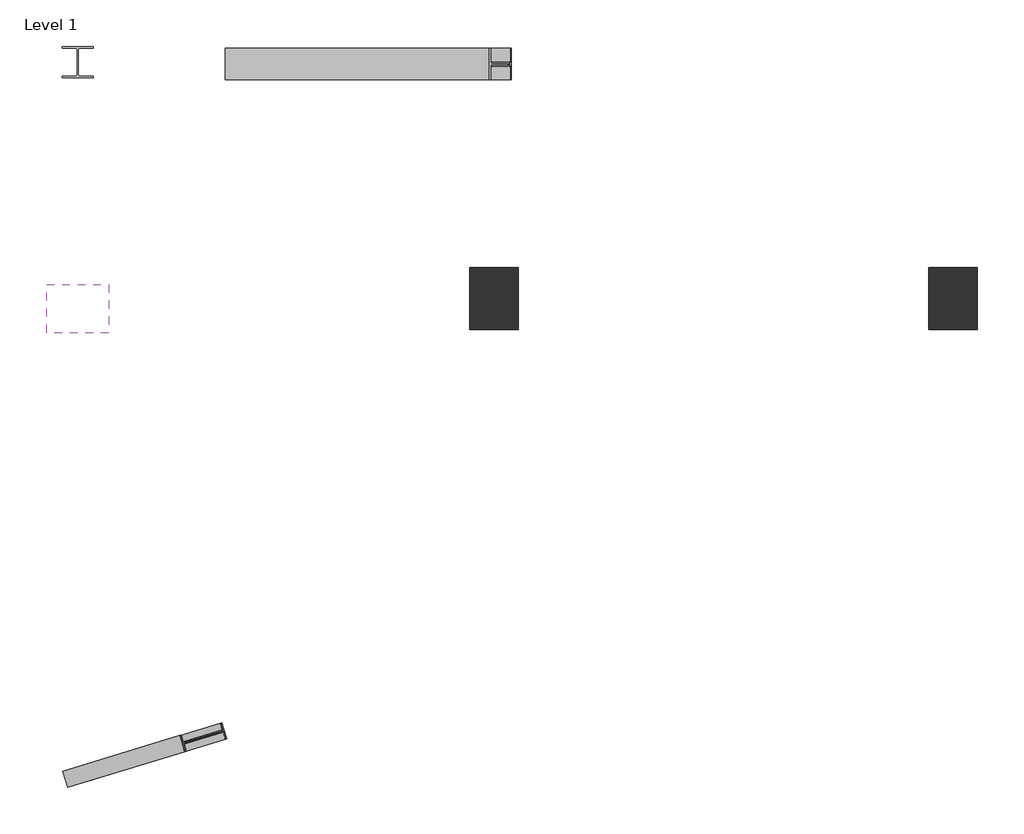
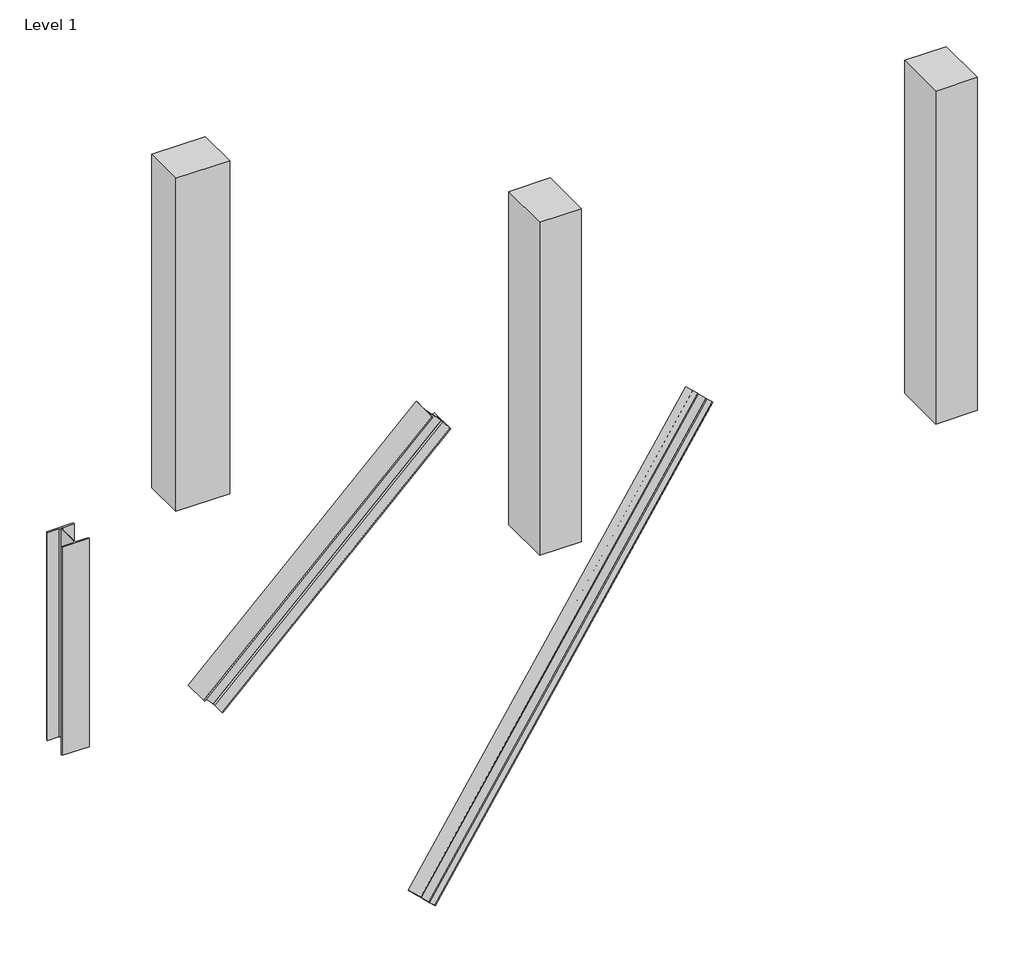
# One storey: 5 columns, 1 beam.
"""IFC4 building model written with IfcOpenShell, lengths in millimetres."""

import ifcopenshell
import ifcopenshell.guid

model = None  # the IFC model being written
_history = None  # IfcOwnerHistory: only IFC2X3 demands one
_inside = {}  # id of a spatial element -> (the spatial element, [elements in it])
_under = {}  # id of a project, library or spatial element -> (it, [spatial elements below it])
_declared = {}  # id of a project -> (the project, [libraries it declares])
_typed = {}  # id of a type object -> (the type object, [elements of that type])
_made_of = {}  # id of a material, layer set ... -> (it, [elements and type objects made of it])


def new_model(schema):
    """Start an empty IFC model of exactly this schema.

    Asked for "IFC4X3", IfcOpenShell would pick the latest addendum, in which some entities
    have other attributes; the version numbers below select the first issue.
    IFC2X3 requires an IfcOwnerHistory on every rooted entity: one is made here for all.
    """
    global model, _history
    if schema == "IFC4X3":
        model = ifcopenshell.file(schema_version=(4, 3, 0, 0))
    else:
        model = ifcopenshell.file(schema=schema)
    _inside.clear()
    _under.clear()
    _declared.clear()
    _typed.clear()
    _made_of.clear()
    _history = None
    if model.schema == "IFC2X3":
        org = make("IfcOrganization", Name="unknown")
        user = make(
            "IfcPersonAndOrganization",
            ThePerson=make("IfcPerson", FamilyName="unknown"),
            TheOrganization=org,
        )
        app = make(
            "IfcApplication",
            ApplicationDeveloper=org,
            Version="unknown",
            ApplicationFullName="unknown",
            ApplicationIdentifier="unknown",
        )
        _history = make(
            "IfcOwnerHistory",
            OwningUser=user,
            OwningApplication=app,
            ChangeAction="ADDED",
            CreationDate=0,
        )
    return model


def make(cls, **values):
    """One entity of the class cls with the attributes given. An attribute that is None is left unset."""
    return model.create_entity(
        cls, **{name: value for name, value in values.items() if value is not None}
    )


def rooted(cls, **values):
    """An entity with a GlobalId (a new one), such as an element, a storey or a relation."""
    return make(cls, GlobalId=ifcopenshell.guid.new(), OwnerHistory=_history, **values)


def si_unit(unit_type, name, prefix=None):
    """IfcSIUnit, for example si_unit("LENGTHUNIT", "METRE", prefix="MILLI")."""
    return make("IfcSIUnit", UnitType=unit_type, Prefix=prefix, Name=name)


def assignment(units):
    """IfcUnitAssignment: the units of a project."""
    return None if units is None else make("IfcUnitAssignment", Units=units)


def point(xyz):
    """IfcCartesianPoint."""
    return None if xyz is None else make("IfcCartesianPoint", Coordinates=xyz)


def direction(xyz):
    """IfcDirection."""
    return None if xyz is None else make("IfcDirection", DirectionRatios=xyz)


def frame(location, z_axis=None, x_axis=None):
    """IfcAxis2Placement3D, a coordinate frame: its origin and axes. An axis left out is left unset."""
    return make(
        "IfcAxis2Placement3D",
        Location=point(location),
        Axis=direction(z_axis),
        RefDirection=direction(x_axis),
    )


def frame_2d(location, x_axis=None):
    """IfcAxis2Placement2D, a coordinate frame in the plane: its origin and x axis."""
    return make(
        "IfcAxis2Placement2D", Location=point(location), RefDirection=direction(x_axis)
    )


def origin():
    """The frame at (0, 0, 0) with its axes left unset."""
    return frame((0.0, 0.0, 0.0))


def origin_with_axes():
    """The frame at (0, 0, 0) with the z axis (0, 0, 1) and the x axis (1, 0, 0) written out."""
    return frame((0.0, 0.0, 0.0), z_axis=(0.0, 0.0, 1.0), x_axis=(1.0, 0.0, 0.0))


def place(relative_to, where):
    """IfcLocalPlacement: puts the frame where relative to a parent placement (None: the world)."""
    return make(
        "IfcLocalPlacement", PlacementRelTo=relative_to, RelativePlacement=where
    )


def context(
    kind, dimensions, precision=None, world=None, true_north=None, identifier=None
):
    """IfcGeometricRepresentationContext, for example the 3D "Model" context."""
    return make(
        "IfcGeometricRepresentationContext",
        ContextIdentifier=identifier,
        ContextType=kind,
        CoordinateSpaceDimension=dimensions,
        Precision=precision,
        WorldCoordinateSystem=world,
        TrueNorth=true_north,
    )


def project(units=None, contexts=None):
    """IfcProject with its units and contexts."""
    return rooted(
        "IfcProject",
        Name="project",
        RepresentationContexts=contexts,
        UnitsInContext=assignment(units),
    )


def spatial(cls, under=None, at=None, **own):
    """A site, building, storey or space (cls), placed at a placement, below another one or the project."""
    s = rooted(cls, ObjectPlacement=at, **own)
    if under is not None:
        _under.setdefault(under.id(), (under, []))[1].append(s)
    return s


def polyline(points):
    """IfcPolyline through the points."""
    return make("IfcPolyline", Points=[point(p) for p in points])


def circle_curve(where, radius):
    """IfcCircle in the frame where."""
    return make("IfcCircle", Position=where, Radius=radius)


def trimmed(basis, trim1, trim2, sense, master):
    """IfcTrimmedCurve: the piece of a basis curve between two trims."""
    return make(
        "IfcTrimmedCurve",
        BasisCurve=basis,
        Trim1=trim1,
        Trim2=trim2,
        SenseAgreement=sense,
        MasterRepresentation=master,
    )


def segment(curve, same_sense, transition):
    """IfcCompositeCurveSegment."""
    return make(
        "IfcCompositeCurveSegment",
        Transition=transition,
        SameSense=same_sense,
        ParentCurve=curve,
    )


def composite_curve(segments, self_intersect=None):
    """IfcCompositeCurve: segments joined end to end."""
    return make("IfcCompositeCurve", Segments=segments, SelfIntersect=self_intersect)


def outline(outer, holes=None, kind="AREA"):
    """IfcArbitraryClosedProfileDef: a profile drawn as a closed curve; with holes, ...WithVoids."""
    if holes is None:
        return make("IfcArbitraryClosedProfileDef", ProfileType=kind, OuterCurve=outer)
    return make(
        "IfcArbitraryProfileDefWithVoids",
        ProfileType=kind,
        OuterCurve=outer,
        InnerCurves=holes,
    )


def extrude(swept, where, along, depth):
    """IfcExtrudedAreaSolid: the profile swept, set in the frame where, extruded along a direction by depth."""
    return make(
        "IfcExtrudedAreaSolid",
        SweptArea=swept,
        Position=where,
        ExtrudedDirection=direction(along),
        Depth=depth,
    )


def shape(context_of_items, identifier, shape_type, items):
    """IfcShapeRepresentation: the items that make up one representation, for example the "Body"."""
    return make(
        "IfcShapeRepresentation",
        ContextOfItems=context_of_items,
        RepresentationIdentifier=identifier,
        RepresentationType=shape_type,
        Items=items,
    )


def source(mapping_origin, context_of_items, identifier, shape_type, items):
    """IfcRepresentationMap: a shape defined once, which mapped items show again and again."""
    return make(
        "IfcRepresentationMap",
        MappingOrigin=mapping_origin,
        MappedRepresentation=shape(context_of_items, identifier, shape_type, items),
    )


def transform(
    local_origin,
    x_axis=None,
    y_axis=None,
    z_axis=None,
    scale=None,
    scale2=None,
    scale3=None,
    uniform=True,
):
    """IfcCartesianTransformationOperator3D, or its non-uniform kind. x_axis, y_axis, z_axis: its Axis1, 2, 3."""
    if uniform:
        return make(
            "IfcCartesianTransformationOperator3D",
            Axis1=direction(x_axis),
            Axis2=direction(y_axis),
            LocalOrigin=point(local_origin),
            Scale=scale,
            Axis3=direction(z_axis),
        )
    return make(
        "IfcCartesianTransformationOperator3DnonUniform",
        Axis1=direction(x_axis),
        Axis2=direction(y_axis),
        LocalOrigin=point(local_origin),
        Scale=scale,
        Axis3=direction(z_axis),
        Scale2=scale2,
        Scale3=scale3,
    )


def mapped(mapping_source, mapping_target):
    """IfcMappedItem: shows the shape of a source again, moved by a transform."""
    return make(
        "IfcMappedItem", MappingSource=mapping_source, MappingTarget=mapping_target
    )


def made_of(thing, what):
    """Note that an element or type object is made of a material, layer set ...; save() writes the relation."""
    if what is not None:
        _made_of.setdefault(what.id(), (what, []))[1].append(thing)
    return thing


def element(
    cls,
    number,
    at=None,
    inside=None,
    cuts=None,
    type_object=None,
    material=None,
    context=None,
    identifier="Body",
    shape_type=None,
    held_by="IfcProductDefinitionShape",
    body=None,
    shapes=None,
    **own,
):
    """One element of the class cls, such as IfcWall. Its Tag is "e" and its number.

    at: its placement. inside: the storey or other place that contains it. cuts: it is an
    opening in that element (IfcRelVoidsElement). A single representation is given by context,
    identifier, shape_type and body (its items); several are given by shapes. held_by: the class
    of the entity that holds the representations. save() writes the other relations.
    """
    e = rooted(cls, Tag="e%d" % number, ObjectPlacement=at, **own)
    if body is not None:
        shapes = [shape(context, identifier, shape_type, body)]
    if shapes is not None:
        e.Representation = make(held_by, Representations=shapes)
    if inside is not None:
        _inside.setdefault(inside.id(), (inside, []))[1].append(e)
    if cuts is not None:
        rooted(
            "IfcRelVoidsElement", RelatingBuildingElement=cuts, RelatedOpeningElement=e
        )
    if type_object is not None:
        _typed.setdefault(type_object.id(), (type_object, []))[1].append(e)
    return made_of(e, material)


def aggregate(whole, parts):
    """IfcRelAggregates: a whole, such as a stair, and the parts it consists of."""
    return rooted("IfcRelAggregates", RelatingObject=whole, RelatedObjects=parts)


def save(model, path):
    """Write the relations noted so far, then the file.

    IfcRelAggregates (storeys below a building ...), IfcRelContainedInSpatialStructure (elements
    in a storey), IfcRelDefinesByType, IfcRelAssociatesMaterial and IfcRelDeclares: one each for
    every whole, place, type object, material and project.
    """
    for whole, parts in _under.values():
        aggregate(whole, parts)
    for where, things in _inside.values():
        rooted(
            "IfcRelContainedInSpatialStructure",
            RelatedElements=things,
            RelatingStructure=where,
        )
    for kind, things in _typed.values():
        rooted("IfcRelDefinesByType", RelatedObjects=things, RelatingType=kind)
    for what, things in _made_of.values():
        rooted("IfcRelAssociatesMaterial", RelatedObjects=things, RelatingMaterial=what)
    for by, libraries in _declared.values():
        rooted("IfcRelDeclares", RelatingContext=by, RelatedDefinitions=libraries)
    model.write(path)


def ub_universal_beams_ub305x165x40_d3799931(model_context):
    return source(origin(), model_context, "Body", "SweptSolid", [
        extrude(outline(composite_curve([segment(polyline([(82.5, -141.5), (82.5, -151.7), (-82.5, -151.7), (-82.5, -141.5), (-11.9, -141.5)]), True, "CONTINUOUS"), segment(trimmed(circle_curve(frame_2d((-11.9, -132.6)), 8.9), [point((-11.9, -141.5))], [point((-3.0, -132.6))], True, "CARTESIAN"), True, "CONTINUOUS"), segment(polyline([(-3.0, -132.6), (-3.0, 132.6)]), True, "CONTINUOUS"), segment(trimmed(circle_curve(frame_2d((-11.9, 132.6)), 8.9), [point((-3.0, 132.6))], [point((-11.9, 141.5))], True, "CARTESIAN"), True, "CONTINUOUS"), segment(polyline([(-11.9, 141.5), (-82.5, 141.5), (-82.5, 151.7), (82.5, 151.7), (82.5, 141.5), (11.9, 141.5)]), True, "CONTINUOUS"), segment(trimmed(circle_curve(frame_2d((11.9, 132.6)), 8.9), [point((11.9, 141.5))], [point((3.0, 132.6))], True, "CARTESIAN"), True, "CONTINUOUS"), segment(polyline([(3.0, 132.6), (3.0, -132.6)]), True, "CONTINUOUS"), segment(trimmed(circle_curve(frame_2d((11.9, -132.6)), 8.9), [point((3.0, -132.6))], [point((11.9, -141.5))], True, "CARTESIAN"), True, "CONTINUOUS"), segment(polyline([(11.9, -141.5), (82.5, -141.5)]), True, "CONTINUOUS")], self_intersect=False)), frame((-2828.4, 0.0, 0.0), z_axis=(1.0, 0.0, 0.0), x_axis=(0.0, 1.0, 0.0)), (0.0, 0.0, 1.0), 5656.8),
    ])


def m_rectangular_column_475_x_610mm_b7c60445(model_context):
    return source(origin(), model_context, "Body", "SweptSolid", [
        extrude(outline(polyline([(305.0, 237.5), (305.0, -237.5), (-305.0, -237.5), (-305.0, 237.5), (305.0, 237.5)])), origin_with_axes(), (0.0, 0.0, 1.0), 4000.0),
    ])


def m_rectangular_column_475_x_610mm_e62a7db6(model_context):
    return source(origin(), model_context, "Body", "SweptSolid", [
        extrude(outline(polyline([(305.0, 237.5), (305.0, -237.5), (-305.0, -237.5), (-305.0, 237.5), (305.0, 237.5)])), frame((0.0, 0.0, 2000.0), z_axis=(0.0, 0.0, 1.0), x_axis=(1.0, 0.0, 0.0)), (0.0, 0.0, 1.0), 4000.0),
    ])


def uc_universal_columns_column_uc305x305x97_2af35403(model_context):
    return source(origin(), model_context, "Body", "SweptSolid", [
        extrude(outline(composite_curve([segment(polyline([(152.65, 153.95), (152.65, 138.55), (20.15, 138.55)]), True, "CONTINUOUS"), segment(trimmed(circle_curve(frame_2d((20.15, 123.35)), 15.2), [point((20.15, 138.55))], [point((4.95, 123.35))], True, "CARTESIAN"), True, "CONTINUOUS"), segment(polyline([(4.95, 123.35), (4.95, -123.35)]), True, "CONTINUOUS"), segment(trimmed(circle_curve(frame_2d((20.15, -123.35)), 15.2), [point((4.95, -123.35))], [point((20.15, -138.55))], True, "CARTESIAN"), True, "CONTINUOUS"), segment(polyline([(20.15, -138.55), (152.65, -138.55), (152.65, -153.95), (-152.65, -153.95), (-152.65, -138.55), (-20.15, -138.55)]), True, "CONTINUOUS"), segment(trimmed(circle_curve(frame_2d((-20.15, -123.35)), 15.2), [point((-20.15, -138.55))], [point((-4.95, -123.35))], True, "CARTESIAN"), True, "CONTINUOUS"), segment(polyline([(-4.95, -123.35), (-4.95, 123.35)]), True, "CONTINUOUS"), segment(trimmed(circle_curve(frame_2d((-20.15, 123.35)), 15.2), [point((-4.95, 123.35))], [point((-20.15, 138.55))], True, "CARTESIAN"), True, "CONTINUOUS"), segment(polyline([(-20.15, 138.55), (-152.65, 138.55), (-152.65, 153.95), (152.65, 153.95)]), True, "CONTINUOUS")], self_intersect=False)), frame((0.0, 0.0, -2500.0), z_axis=(0.0, 0.0, 1.0), x_axis=(1.0, 0.0, 0.0)), (0.0, 0.0, 1.0), 2500.0),
    ])


model = new_model("IFC4")

# Units and contexts
model_context = context("Model", 3, world=origin())
ifc_project = project(units=[si_unit("LENGTHUNIT", "METRE", prefix="MILLI")], contexts=[model_context])

# Site, building, storey
site = spatial("IfcSite", under=ifc_project)
building = spatial("IfcBuilding", under=site)
storey = spatial("IfcBuildingStorey", under=building, Name="Level 1", Elevation=0.0)

# Beam
placement = place(None, origin())
ub_universal_beams_ub305x165x40_shape = ub_universal_beams_ub305x165x40_d3799931(model_context)
element("IfcBeam", 1, ObjectType="UB-Universal Beams : UB305x165x40", at=placement, inside=storey, context=model_context, shape_type="MappedRepresentation", body=[
    mapped(ub_universal_beams_ub305x165x40_shape, transform((-13362.6939033, 6195.0671002, 1892.7319013), x_axis=(-0.6762095778224118, -0.20673801503650877, -0.7071067811865475), y_axis=(0.29237170472272356, -0.9563047559630395, 0.0), z_axis=(-0.6762095778224118, -0.2067380150365088, 0.7071067811865475))),
])

# Columns
m_rectangular_column_475_x_610mm_shape = m_rectangular_column_475_x_610mm_b7c60445(model_context)
element("IfcColumn", 2, ObjectType="M_Rectangular Column : 475 x 610mm", at=placement, inside=storey, context=model_context, shape_type="MappedRepresentation", body=[
    mapped(m_rectangular_column_475_x_610mm_shape, transform((-11172.9587266, 10295.0671002, 0.0), x_axis=(0.0, 1.0, 0.0), y_axis=(-1.0, 0.0, 0.0), z_axis=(0.0, 0.0, 1.0))),
])
m_rectangular_column_475_x_610mm_2_shape = m_rectangular_column_475_x_610mm_e62a7db6(model_context)
element("IfcColumn", 3, ObjectType="M_Rectangular Column : 475 x 610mm", at=placement, inside=storey, context=model_context, shape_type="MappedRepresentation", body=[
    mapped(m_rectangular_column_475_x_610mm_2_shape, transform((-15255.4258046, 10195.0671002, 0.0), x_axis=(1.0, 0.0, 0.0), y_axis=(0.0, 1.0, 0.0), z_axis=(0.0, 0.0, 1.0))),
])
element("IfcColumn", 4, ObjectType="M_Rectangular Column : 475 x 610mm", at=placement, inside=storey, context=model_context, shape_type="MappedRepresentation", body=[
    mapped(m_rectangular_column_475_x_610mm_shape, transform((-6672.9587266, 10295.0671002, 0.0), x_axis=(0.0, 1.0, 0.0), y_axis=(-1.0, 0.0, 0.0), z_axis=(0.0, 0.0, 1.0))),
])
element("IfcColumn", 5, ObjectType="UC-Universal Columns-Column : UC305x305x97", at=placement, inside=storey, context=model_context, shape_type="SweptSolid", body=[
    extrude(outline(composite_curve([segment(polyline([(305.3, 0.0), (305.3, -15.4), (172.8, -15.4)]), True, "CONTINUOUS"), segment(trimmed(circle_curve(frame_2d((172.8, -30.6)), 15.2), [point((172.8, -15.4))], [point((157.6, -30.6))], True, "CARTESIAN"), True, "CONTINUOUS"), segment(polyline([(157.6, -30.6), (157.6, -277.3000001)]), True, "CONTINUOUS"), segment(trimmed(circle_curve(frame_2d((172.8, -277.3000001)), 15.2), [point((157.6, -277.3000001))], [point((172.8, -292.5))], True, "CARTESIAN"), True, "CONTINUOUS"), segment(polyline([(172.8, -292.5), (305.3, -292.5), (305.3, -307.9), (0.0, -307.9), (0.0, -292.5), (132.5, -292.5)]), True, "CONTINUOUS"), segment(trimmed(circle_curve(frame_2d((132.5, -277.3000001)), 15.2), [point((132.5, -292.5))], [point((147.7, -277.3000001))], True, "CARTESIAN"), True, "CONTINUOUS"), segment(polyline([(147.7, -277.3000001), (147.7, -30.6)]), True, "CONTINUOUS"), segment(trimmed(circle_curve(frame_2d((132.5, -30.6)), 15.2), [point((147.7, -30.6))], [point((132.5, -15.4))], True, "CARTESIAN"), True, "CONTINUOUS"), segment(polyline([(132.5, -15.4), (0.0, -15.4), (0.0, 0.0), (305.3, 0.0)]), True, "CONTINUOUS")], self_intersect=False)), frame((-13809.4065724, 12442.4171002, -2389.2258433), z_axis=(0.7195463248327014, 0.0, 0.6944444444444441), x_axis=(0.0, 1.0, 0.0)), (0.0, 0.0, 1.0), 3600.0),
])
uc_universal_columns_column_uc305x305x97_shape = uc_universal_columns_column_uc305x305x97_2af35403(model_context)
element("IfcColumn", 6, ObjectType="UC-Universal Columns-Column : UC305x305x97", at=placement, inside=storey, context=model_context, shape_type="MappedRepresentation", body=[
    mapped(uc_universal_columns_column_uc305x305x97_shape, transform((-15255.4258046, 12612.4709614, 0.0), x_axis=(1.0, 0.0, 0.0), y_axis=(0.0, 1.0, 0.0), z_axis=(0.0, 0.0, 1.0))),
])

save(model, "model.ifc")

# Revit data of these elements
# Project information
#   Project Issue Date = "Issue Date"
#   Project Status = "Project Status"
#   Client Name = "Owner"
#   Project Address = "Enter address here"
#   Project Name = "Project Name"
#   Project Number = "0001"
# Type "UB-Universal Beams : UB305x165x40"
#   Section Name Key = "UB305X165X40"
#   Width = 16.5 cm
#   Web Thickness = 0.6 cm
#   Web Fillet = 0.89 cm
#   Warping Constant = 164000.0 cm⁶
#   Torsional Moment of Inertia = 14.70 cm⁴
#   Section Area = 51.3 cm²
#   Plastic Modulus weak axis = 142.0 cm³
#   Plastic Modulus strong axis = 623.0 cm³
#   Nominal Weight = 40.2999 kgf/m
#   Moment of Inertia weak axis = 764.00 cm⁴
#   Moment of Inertia strong axis = 8503.00 cm⁴
#   Height = 30.34 cm
#   Flange Thickness = 1.02 cm
#   Elastic Modulus weak axis = 92.6 cm³
#   Elastic Modulus strong axis = 560.0 cm³
#   Centroid Vertical = 15.17 cm
#   Centroid Horizontal = 8.25 cm
#   Bolt Spacing = 9.0 cm
#   Length [instance default] = 1500 mm
#   Structural Material [instance default] = Metal - Steel 43-275
#   Type Comments = ""
#   Assembly Code = ""
# Type "M_Rectangular Column : 475 x 610mm"
#   Depth = 475 mm
#   Offset Base = 0 mm
#   Offset Top = 0 mm
#   Width = 610 mm
#   Material = none
# Type "UC-Universal Columns-Column : UC305x305x97"
#   Section Name Key = "UC305x305x97"
#   Width = 30.53 cm
#   Web Thickness = 0.99 cm
#   Web Fillet = 1.52 cm
#   Warping Constant = 1560000.0 cm⁶
#   Torsional Moment of Inertia = 91.20 cm⁴
#   Section Area = 123.0 cm²
#   Plastic Modulus weak axis = 726.0 cm³
#   Plastic Modulus strong axis = 1592.0 cm³
#   Nominal Weight = 96.8996 kgf/m
#   Moment of Inertia weak axis = 7308.00 cm⁴
#   Moment of Inertia strong axis = 22249.00 cm⁴
#   Height = 30.79 cm
#   Flange Thickness = 1.54 cm
#   Elastic Modulus weak axis = 479.0 cm³
#   Elastic Modulus strong axis = 1445.0 cm³
#   Centroid Vertical = 15.395 cm
#   Centroid Horizontal = 15.265 cm
#   Bolt Spacing = 14.0 cm
#   Structural Material [instance default] = Metal - Steel 43-275
#   Type Comments = ""
#   Assembly Code = ""
# Element 1 (IfcBeam, "UB-Universal Beams : UB305x165x40")
#   Structural Material = Metal - Steel 43-275
#   Phase Created = New Construction
#   Materials on its faces: "Metal - Steel 43-275"
# Elements 2, 3, 4 (IfcColumn, "M_Rectangular Column : 475 x 610mm")
#   Phase Created = New Construction
# Elements 5, 6 (IfcColumn, "UC-Universal Columns-Column : UC305x305x97")
#   Structural Material = Metal - Steel 43-275
#   Phase Created = New Construction
#   Materials on its faces: "Metal - Steel 43-275"
# Materials
#   "Metal - Steel 43-275": class "Metal", colour RGB 247 247 247, transparency 0, Cost = 0
